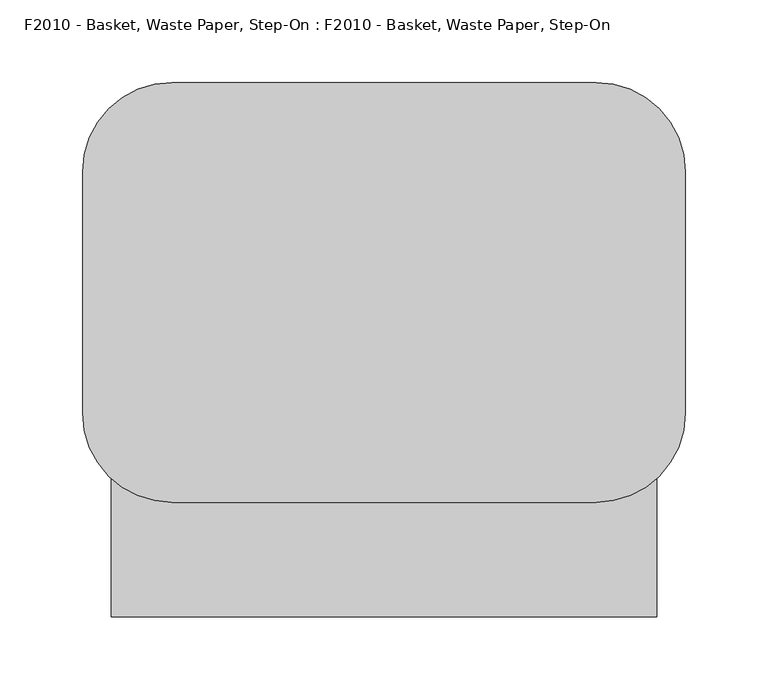
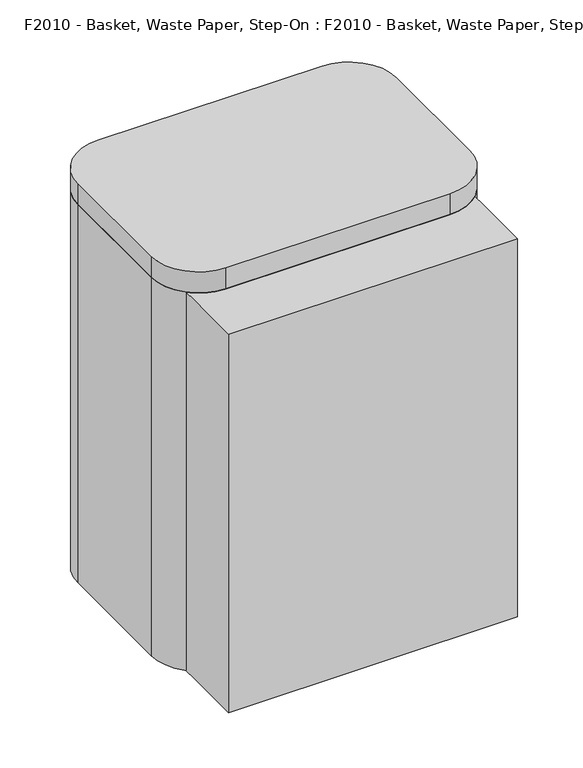
"""IFC4 building model written with IfcOpenShell, lengths in millimetres: proxy geometry, F2010 - Basket, Waste Paper, Step-On : F2010 - Basket, Waste Paper, Step-On."""

import ifcopenshell
import ifcopenshell.guid

model = None  # the IFC model being written
_history = None  # IfcOwnerHistory: only IFC2X3 demands one
_inside = {}  # id of a spatial element -> (the spatial element, [elements in it])
_under = {}  # id of a project, library or spatial element -> (it, [spatial elements below it])
_declared = {}  # id of a project -> (the project, [libraries it declares])
_typed = {}  # id of a type object -> (the type object, [elements of that type])
_made_of = {}  # id of a material, layer set ... -> (it, [elements and type objects made of it])


def new_model(schema):
    """Start an empty IFC model of exactly this schema.

    Asked for "IFC4X3", IfcOpenShell would pick the latest addendum, in which some entities
    have other attributes; the version numbers below select the first issue.
    IFC2X3 requires an IfcOwnerHistory on every rooted entity: one is made here for all.
    """
    global model, _history
    if schema == "IFC4X3":
        model = ifcopenshell.file(schema_version=(4, 3, 0, 0))
    else:
        model = ifcopenshell.file(schema=schema)
    _inside.clear()
    _under.clear()
    _declared.clear()
    _typed.clear()
    _made_of.clear()
    _history = None
    if model.schema == "IFC2X3":
        org = make("IfcOrganization", Name="unknown")
        user = make(
            "IfcPersonAndOrganization",
            ThePerson=make("IfcPerson", FamilyName="unknown"),
            TheOrganization=org,
        )
        app = make(
            "IfcApplication",
            ApplicationDeveloper=org,
            Version="unknown",
            ApplicationFullName="unknown",
            ApplicationIdentifier="unknown",
        )
        _history = make(
            "IfcOwnerHistory",
            OwningUser=user,
            OwningApplication=app,
            ChangeAction="ADDED",
            CreationDate=0,
        )
    return model


def make(cls, **values):
    """One entity of the class cls with the attributes given. An attribute that is None is left unset."""
    return model.create_entity(
        cls, **{name: value for name, value in values.items() if value is not None}
    )


def rooted(cls, **values):
    """An entity with a GlobalId (a new one), such as an element, a storey or a relation."""
    return make(cls, GlobalId=ifcopenshell.guid.new(), OwnerHistory=_history, **values)


def si_unit(unit_type, name, prefix=None):
    """IfcSIUnit, for example si_unit("LENGTHUNIT", "METRE", prefix="MILLI")."""
    return make("IfcSIUnit", UnitType=unit_type, Prefix=prefix, Name=name)


def assignment(units):
    """IfcUnitAssignment: the units of a project."""
    return None if units is None else make("IfcUnitAssignment", Units=units)


def point(xyz):
    """IfcCartesianPoint."""
    return None if xyz is None else make("IfcCartesianPoint", Coordinates=xyz)


def direction(xyz):
    """IfcDirection."""
    return None if xyz is None else make("IfcDirection", DirectionRatios=xyz)


def frame(location, z_axis=None, x_axis=None):
    """IfcAxis2Placement3D, a coordinate frame: its origin and axes. An axis left out is left unset."""
    return make(
        "IfcAxis2Placement3D",
        Location=point(location),
        Axis=direction(z_axis),
        RefDirection=direction(x_axis),
    )


def frame_2d(location, x_axis=None):
    """IfcAxis2Placement2D, a coordinate frame in the plane: its origin and x axis."""
    return make(
        "IfcAxis2Placement2D", Location=point(location), RefDirection=direction(x_axis)
    )


def origin():
    """The frame at (0, 0, 0) with its axes left unset."""
    return frame((0.0, 0.0, 0.0))


def origin_with_axes():
    """The frame at (0, 0, 0) with the z axis (0, 0, 1) and the x axis (1, 0, 0) written out."""
    return frame((0.0, 0.0, 0.0), z_axis=(0.0, 0.0, 1.0), x_axis=(1.0, 0.0, 0.0))


def place(relative_to, where):
    """IfcLocalPlacement: puts the frame where relative to a parent placement (None: the world)."""
    return make(
        "IfcLocalPlacement", PlacementRelTo=relative_to, RelativePlacement=where
    )


def context(
    kind, dimensions, precision=None, world=None, true_north=None, identifier=None
):
    """IfcGeometricRepresentationContext, for example the 3D "Model" context."""
    return make(
        "IfcGeometricRepresentationContext",
        ContextIdentifier=identifier,
        ContextType=kind,
        CoordinateSpaceDimension=dimensions,
        Precision=precision,
        WorldCoordinateSystem=world,
        TrueNorth=true_north,
    )


def project(units=None, contexts=None):
    """IfcProject with its units and contexts."""
    return rooted(
        "IfcProject",
        Name="project",
        RepresentationContexts=contexts,
        UnitsInContext=assignment(units),
    )


def spatial(cls, under=None, at=None, **own):
    """A site, building, storey or space (cls), placed at a placement, below another one or the project."""
    s = rooted(cls, ObjectPlacement=at, **own)
    if under is not None:
        _under.setdefault(under.id(), (under, []))[1].append(s)
    return s


def polyline(points):
    """IfcPolyline through the points."""
    return make("IfcPolyline", Points=[point(p) for p in points])


def circle_curve(where, radius):
    """IfcCircle in the frame where."""
    return make("IfcCircle", Position=where, Radius=radius)


def trimmed(basis, trim1, trim2, sense, master):
    """IfcTrimmedCurve: the piece of a basis curve between two trims."""
    return make(
        "IfcTrimmedCurve",
        BasisCurve=basis,
        Trim1=trim1,
        Trim2=trim2,
        SenseAgreement=sense,
        MasterRepresentation=master,
    )


def segment(curve, same_sense, transition):
    """IfcCompositeCurveSegment."""
    return make(
        "IfcCompositeCurveSegment",
        Transition=transition,
        SameSense=same_sense,
        ParentCurve=curve,
    )


def composite_curve(segments, self_intersect=None):
    """IfcCompositeCurve: segments joined end to end."""
    return make("IfcCompositeCurve", Segments=segments, SelfIntersect=self_intersect)


def outline(outer, holes=None, kind="AREA"):
    """IfcArbitraryClosedProfileDef: a profile drawn as a closed curve; with holes, ...WithVoids."""
    if holes is None:
        return make("IfcArbitraryClosedProfileDef", ProfileType=kind, OuterCurve=outer)
    return make(
        "IfcArbitraryProfileDefWithVoids",
        ProfileType=kind,
        OuterCurve=outer,
        InnerCurves=holes,
    )


def extrude(swept, where, along, depth):
    """IfcExtrudedAreaSolid: the profile swept, set in the frame where, extruded along a direction by depth."""
    return make(
        "IfcExtrudedAreaSolid",
        SweptArea=swept,
        Position=where,
        ExtrudedDirection=direction(along),
        Depth=depth,
    )


def shape(context_of_items, identifier, shape_type, items):
    """IfcShapeRepresentation: the items that make up one representation, for example the "Body"."""
    return make(
        "IfcShapeRepresentation",
        ContextOfItems=context_of_items,
        RepresentationIdentifier=identifier,
        RepresentationType=shape_type,
        Items=items,
    )


def source(mapping_origin, context_of_items, identifier, shape_type, items):
    """IfcRepresentationMap: a shape defined once, which mapped items show again and again."""
    return make(
        "IfcRepresentationMap",
        MappingOrigin=mapping_origin,
        MappedRepresentation=shape(context_of_items, identifier, shape_type, items),
    )


def transform(
    local_origin,
    x_axis=None,
    y_axis=None,
    z_axis=None,
    scale=None,
    scale2=None,
    scale3=None,
    uniform=True,
):
    """IfcCartesianTransformationOperator3D, or its non-uniform kind. x_axis, y_axis, z_axis: its Axis1, 2, 3."""
    if uniform:
        return make(
            "IfcCartesianTransformationOperator3D",
            Axis1=direction(x_axis),
            Axis2=direction(y_axis),
            LocalOrigin=point(local_origin),
            Scale=scale,
            Axis3=direction(z_axis),
        )
    return make(
        "IfcCartesianTransformationOperator3DnonUniform",
        Axis1=direction(x_axis),
        Axis2=direction(y_axis),
        LocalOrigin=point(local_origin),
        Scale=scale,
        Axis3=direction(z_axis),
        Scale2=scale2,
        Scale3=scale3,
    )


def mapped(mapping_source, mapping_target):
    """IfcMappedItem: shows the shape of a source again, moved by a transform."""
    return make(
        "IfcMappedItem", MappingSource=mapping_source, MappingTarget=mapping_target
    )


def made_of(thing, what):
    """Note that an element or type object is made of a material, layer set ...; save() writes the relation."""
    if what is not None:
        _made_of.setdefault(what.id(), (what, []))[1].append(thing)
    return thing


def element(
    cls,
    number,
    at=None,
    inside=None,
    cuts=None,
    type_object=None,
    material=None,
    context=None,
    identifier="Body",
    shape_type=None,
    held_by="IfcProductDefinitionShape",
    body=None,
    shapes=None,
    **own,
):
    """One element of the class cls, such as IfcWall. Its Tag is "e" and its number.

    at: its placement. inside: the storey or other place that contains it. cuts: it is an
    opening in that element (IfcRelVoidsElement). A single representation is given by context,
    identifier, shape_type and body (its items); several are given by shapes. held_by: the class
    of the entity that holds the representations. save() writes the other relations.
    """
    e = rooted(cls, Tag="e%d" % number, ObjectPlacement=at, **own)
    if body is not None:
        shapes = [shape(context, identifier, shape_type, body)]
    if shapes is not None:
        e.Representation = make(held_by, Representations=shapes)
    if inside is not None:
        _inside.setdefault(inside.id(), (inside, []))[1].append(e)
    if cuts is not None:
        rooted(
            "IfcRelVoidsElement", RelatingBuildingElement=cuts, RelatedOpeningElement=e
        )
    if type_object is not None:
        _typed.setdefault(type_object.id(), (type_object, []))[1].append(e)
    return made_of(e, material)


def aggregate(whole, parts):
    """IfcRelAggregates: a whole, such as a stair, and the parts it consists of."""
    return rooted("IfcRelAggregates", RelatingObject=whole, RelatedObjects=parts)


def save(model, path):
    """Write the relations noted so far, then the file.

    IfcRelAggregates (storeys below a building ...), IfcRelContainedInSpatialStructure (elements
    in a storey), IfcRelDefinesByType, IfcRelAssociatesMaterial and IfcRelDeclares: one each for
    every whole, place, type object, material and project.
    """
    for whole, parts in _under.values():
        aggregate(whole, parts)
    for where, things in _inside.values():
        rooted(
            "IfcRelContainedInSpatialStructure",
            RelatedElements=things,
            RelatingStructure=where,
        )
    for kind, things in _typed.values():
        rooted("IfcRelDefinesByType", RelatedObjects=things, RelatingType=kind)
    for what, things in _made_of.values():
        rooted("IfcRelAssociatesMaterial", RelatedObjects=things, RelatingMaterial=what)
    for by, libraries in _declared.values():
        rooted("IfcRelDeclares", RelatingContext=by, RelatedDefinitions=libraries)
    model.write(path)


def plane_surface(at):
    """IfcPlane: the flat surface through the origin of the frame at, square to its z axis."""
    return make("IfcPlane", Position=at)


def cylinder_surface(at, radius):
    """IfcCylindricalSurface: all points at the distance radius from the z axis of the frame at."""
    return make("IfcCylindricalSurface", Position=at, Radius=radius)


def revolved_surface(curve, axis_point, axis_direction):
    """IfcSurfaceOfRevolution: the curve turned about the line through axis_point along axis_direction."""
    return make(
        "IfcSurfaceOfRevolution",
        SweptCurve=make("IfcArbitraryOpenProfileDef", ProfileType="CURVE", Curve=curve),
        AxisPosition=make("IfcAxis1Placement", Location=point(axis_point), Axis=direction(axis_direction)),
    )


def advanced_brep(points, edges, surfaces, faces):
    """IfcAdvancedBrep: a solid bounded by faces that lie on surfaces and meet in shared edges.

    An edge is (start, end): straight between two places in points (the first is 0);
    or (start, end, curve); or (start, end, curve, False) where it runs against its curve.
    A face is (place in surfaces, loops), or (place, loops, False) where it looks against
    its surface's normal. A loop lists edges by number (the first is 1), with a minus sign
    where the edge is run from its end to its start. The first loop is the outer one.
    """
    corners = [point(p) for p in points]
    vertices = [make("IfcVertexPoint", VertexGeometry=c) for c in corners]
    made = []
    for start, end, *more in edges:
        made.append(
            make(
                "IfcEdgeCurve",
                EdgeStart=vertices[start],
                EdgeEnd=vertices[end],
                EdgeGeometry=more[0] if more else make("IfcPolyline", Points=[corners[start], corners[end]]),
                SameSense=more[1] if len(more) > 1 else True,
            )
        )
    hull = []
    for where, loops, *sense in faces:
        bounds = []
        for j, loop in enumerate(loops):
            ring = [make("IfcOrientedEdge", EdgeElement=made[abs(k) - 1], Orientation=k > 0) for k in loop]
            bounds.append(
                make(
                    "IfcFaceOuterBound" if j == 0 else "IfcFaceBound",
                    Bound=make("IfcEdgeLoop", EdgeList=ring),
                    Orientation=True,
                )
            )
        hull.append(make("IfcAdvancedFace", Bounds=bounds, FaceSurface=surfaces[where], SameSense=sense[0] if sense else True))
    return make("IfcAdvancedBrep", Outer=make("IfcClosedShell", CfsFaces=hull))


def f2010_basket_waste_paper_step_on_f2010_basket_waste_paper_f2c5e097(model_context):
    return source(origin(), model_context, "Body", "SolidModel", [
        advanced_brep(
        [(128.266525, 170.9615385, 457.2), (-128.266525, 170.9615385, 457.2), (-182.241525, 116.9865385, 457.2), (-182.241525, -29.0634615, 457.2), (-128.266525, -83.0384615, 457.2), (128.266525, -83.0384615, 457.2), (182.241525, -29.0634615, 457.2), (182.241525, 116.9865385, 457.2), (-114.3, 164.6115385, 457.2), (114.3, 164.6115385, 457.2), (165.1, 113.8115385, 457.2), (165.1, -25.8884615, 457.2), (114.3, -76.6884615, 457.2), (-114.3, -76.6884615, 457.2), (-165.1, -25.8884615, 457.2), (-165.1, 113.8115385, 457.2), (128.266525, 170.9615385, 0.0), (182.241525, 116.9865385, 0.0), (182.241525, -29.0634615, 0.0), (128.266525, -83.0384615, 0.0), (-128.266525, -83.0384615, 0.0), (-182.241525, -29.0634615, 0.0), (-182.241525, 116.9865385, 0.0), (-128.266525, 170.9615385, 0.0), (114.3, 164.6115385, 12.7), (-114.3, 164.6115385, 12.7), (-165.1, 113.8115385, 12.7), (-165.1, -25.8884615, 12.7), (-114.3, -76.6884615, 12.7), (114.3, -76.6884615, 12.7), (165.1, -25.8884615, 12.7), (165.1, 113.8115385, 12.7)],
        [
            (0, 1),
            (1, 2, circle_curve(frame((-128.266525, 116.9865385, 457.2), z_axis=(0.0, 0.0, 1.0), x_axis=(1.0, 0.0, 0.0)), 53.975)),
            (2, 3),
            (3, 4, circle_curve(frame((-128.266525, -29.0634615, 457.2), z_axis=(0.0, 0.0, 1.0), x_axis=(1.0, 0.0, 0.0)), 53.975)),
            (4, 5),
            (5, 6, circle_curve(frame((128.266525, -29.0634615, 457.2), z_axis=(0.0, 0.0, 1.0), x_axis=(1.0, 0.0, 0.0)), 53.975)),
            (6, 7),
            (7, 0, circle_curve(frame((128.266525, 116.9865385, 457.2), z_axis=(0.0, 0.0, 1.0), x_axis=(1.0, 0.0, 0.0)), 53.975)),
            (8, 9),
            (9, 10, circle_curve(frame((114.3, 113.8115385, 457.2), z_axis=(0.0, 0.0, -1.0), x_axis=(1.0, 0.0, 0.0)), 50.8)),
            (10, 11),
            (11, 12, circle_curve(frame((114.3, -25.8884615, 457.2), z_axis=(0.0, 0.0, -1.0), x_axis=(1.0, 0.0, 0.0)), 50.8)),
            (12, 13),
            (13, 14, circle_curve(frame((-114.3, -25.8884615, 457.2), z_axis=(0.0, 0.0, -1.0), x_axis=(1.0, 0.0, 0.0)), 50.8)),
            (14, 15),
            (15, 8, circle_curve(frame((-114.3, 113.8115385, 457.2), z_axis=(0.0, 0.0, -1.0), x_axis=(1.0, 0.0, 0.0)), 50.8)),
            (16, 17, circle_curve(frame((128.266525, 116.9865385, 0.0), z_axis=(0.0, 0.0, -1.0), x_axis=(1.0, 0.0, 0.0)), 53.975)),
            (17, 18),
            (18, 19, circle_curve(frame((128.266525, -29.0634615, 0.0), z_axis=(0.0, 0.0, -1.0), x_axis=(1.0, 0.0, 0.0)), 53.975)),
            (19, 20),
            (20, 21, circle_curve(frame((-128.266525, -29.0634615, 0.0), z_axis=(0.0, 0.0, -1.0), x_axis=(1.0, 0.0, 0.0)), 53.975)),
            (21, 22),
            (22, 23, circle_curve(frame((-128.266525, 116.9865385, 0.0), z_axis=(0.0, 0.0, -1.0), x_axis=(1.0, 0.0, 0.0)), 53.975)),
            (23, 16),
            (0, 16),
            (23, 1),
            (22, 2),
            (21, 3),
            (20, 4),
            (19, 5),
            (18, 6),
            (17, 7),
            (24, 25),
            (25, 26, circle_curve(frame((-114.3, 113.8115385, 12.7), z_axis=(0.0, 0.0, 1.0), x_axis=(1.0, 0.0, 0.0)), 50.8)),
            (26, 27),
            (27, 28, circle_curve(frame((-114.3, -25.8884615, 12.7), z_axis=(0.0, 0.0, 1.0), x_axis=(1.0, 0.0, 0.0)), 50.8)),
            (28, 29),
            (29, 30, circle_curve(frame((114.3, -25.8884615, 12.7), z_axis=(0.0, 0.0, 1.0), x_axis=(1.0, 0.0, 0.0)), 50.8)),
            (30, 31),
            (31, 24, circle_curve(frame((114.3, 113.8115385, 12.7), z_axis=(0.0, 0.0, 1.0), x_axis=(1.0, 0.0, 0.0)), 50.8)),
            (24, 9),
            (8, 25),
            (15, 26),
            (14, 27),
            (13, 28),
            (12, 29),
            (11, 30),
            (10, 31),
        ],
        [
            plane_surface(frame((-182.241525, 170.9615385, 457.2), z_axis=(0.0, 0.0, 1.0), x_axis=(-1.0, 0.0, 0.0))),
            plane_surface(frame((-182.241525, 170.9615385, 0.0), z_axis=(0.0, 0.0, -1.0), x_axis=(1.0, 0.0, 0.0))),
            plane_surface(frame((128.266525, 170.9615385, 457.2), z_axis=(0.0, 1.0, 0.0), x_axis=(0.0, 0.0, -1.0))),
            cylinder_surface(frame((-128.266525, 116.9865385, 0.0), z_axis=(0.0, 0.0, 1.0), x_axis=(1.0, 0.0, 0.0)), 53.975),
            plane_surface(frame((-182.241525, 116.9865385, 457.2), z_axis=(-1.0, 0.0, 0.0), x_axis=(0.0, 0.0, -1.0))),
            cylinder_surface(frame((-128.266525, -29.0634615, 0.0), z_axis=(0.0, 0.0, 1.0), x_axis=(1.0, 0.0, 0.0)), 53.975),
            plane_surface(frame((-128.266525, -83.0384615, 457.2), z_axis=(0.0, -1.0, 0.0), x_axis=(0.0, 0.0, -1.0))),
            cylinder_surface(frame((128.266525, -29.0634615, 0.0), z_axis=(0.0, 0.0, 1.0), x_axis=(1.0, 0.0, 0.0)), 53.975),
            plane_surface(frame((182.241525, -29.0634615, 457.2), z_axis=(1.0, 0.0, 0.0), x_axis=(0.0, 0.0, -1.0))),
            cylinder_surface(frame((128.266525, 116.9865385, 0.0), z_axis=(0.0, 0.0, 1.0), x_axis=(1.0, 0.0, 0.0)), 53.975),
            plane_surface(frame((-125.091525, 164.6115385, 12.7), z_axis=(0.0, 0.0, 1.0), x_axis=(1.0, 0.0, 0.0))),
            plane_surface(frame((114.3, 164.6115385, 457.2), z_axis=(0.0, -1.0, 0.0), x_axis=(0.0, 0.0, -1.0))),
            revolved_surface(polyline([(-63.5, 113.8115385, 457.2), (-63.5, 113.8115385, 12.7)]), (-114.3, 113.8115385, 12.7), (0.0, 0.0, 1.0)),
            plane_surface(frame((-165.1, 113.8115385, 457.2), z_axis=(1.0, 0.0, 0.0), x_axis=(0.0, 0.0, -1.0))),
            revolved_surface(polyline([(-63.5, -25.8884615, 457.2), (-63.5, -25.8884615, 12.7)]), (-114.3, -25.8884615, 12.7), (0.0, 0.0, 1.0)),
            plane_surface(frame((-114.3, -76.6884615, 457.2), z_axis=(0.0, 1.0, 0.0), x_axis=(0.0, 0.0, -1.0))),
            revolved_surface(polyline([(165.1, -25.8884615, 457.2), (165.1, -25.8884615, 12.7)]), (114.3, -25.8884615, 12.7), (0.0, 0.0, 1.0)),
            plane_surface(frame((165.1, -25.8884615, 457.2), z_axis=(-1.0, 0.0, 0.0), x_axis=(0.0, 0.0, -1.0))),
            revolved_surface(polyline([(165.1, 113.8115385, 457.2), (165.1, 113.8115385, 12.7)]), (114.3, 113.8115385, 12.7), (0.0, 0.0, 1.0)),
        ],
        [
            (0, [[1, 2, 3, 4, 5, 6, 7, 8], [9, 10, 11, 12, 13, 14, 15, 16]]),
            (1, [[17, 18, 19, 20, 21, 22, 23, 24]]),
            (2, [[-1, 25, -24, 26]]),
            (3, [[-2, -26, -23, 27]]),
            (4, [[-3, -27, -22, 28]]),
            (5, [[-4, -28, -21, 29]]),
            (6, [[-5, -29, -20, 30]]),
            (7, [[-6, -30, -19, 31]]),
            (8, [[-7, -31, -18, 32]]),
            (9, [[-8, -32, -17, -25]]),
            (10, [[33, 34, 35, 36, 37, 38, 39, 40]]),
            (11, [[-33, 41, -9, 42]]),
            (12, [[-34, -42, -16, 43]]),
            (13, [[-35, -43, -15, 44]]),
            (14, [[-36, -44, -14, 45]]),
            (15, [[-37, -45, -13, 46]]),
            (16, [[-38, -46, -12, 47]]),
            (17, [[-39, -47, -11, 48]]),
            (18, [[-40, -48, -10, -41]]),
        ],
    ),
        extrude(outline(polyline([(50.8, -83.0384615), (-50.8, -83.0384615), (-50.8, -6.8384615), (50.8, -6.8384615), (50.8, -83.0384615)])), origin_with_axes(), (0.0, 0.0, 1.0), 105.5317808),
        extrude(outline(polyline([(38.1, -57.6384615), (38.1, -133.8384615), (-38.1, -133.8384615), (-38.1, -57.6384615), (38.1, -57.6384615)])), origin_with_axes(), (0.0, 0.0, 1.0), 50.8),
        extrude(outline(composite_curve([segment(trimmed(circle_curve(frame_2d((128.266525, 116.9865385)), 53.975), [point((128.266525, 170.9615385))], [point((182.241525, 116.9865385))], False, "CARTESIAN"), True, "CONTINUOUS"), segment(polyline([(182.241525, 116.9865385), (182.241525, -29.0634615)]), True, "CONTINUOUS"), segment(trimmed(circle_curve(frame_2d((128.266525, -29.0634615)), 53.975), [point((182.241525, -29.0634615))], [point((128.266525, -83.0384615))], False, "CARTESIAN"), True, "CONTINUOUS"), segment(polyline([(128.266525, -83.0384615), (-128.266525, -83.0384615)]), True, "CONTINUOUS"), segment(trimmed(circle_curve(frame_2d((-128.266525, -29.0634615)), 53.975), [point((-128.266525, -83.0384615))], [point((-182.241525, -29.0634615))], False, "CARTESIAN"), True, "CONTINUOUS"), segment(polyline([(-182.241525, -29.0634615), (-182.241525, 116.9865385)]), True, "CONTINUOUS"), segment(trimmed(circle_curve(frame_2d((-128.266525, 116.9865385)), 53.975), [point((-182.241525, 116.9865385))], [point((-128.266525, 170.9615385))], False, "CARTESIAN"), True, "CONTINUOUS"), segment(polyline([(-128.266525, 170.9615385), (128.266525, 170.9615385)]), True, "CONTINUOUS")], self_intersect=False)), frame((0.0, 0.0, 457.2), z_axis=(0.0, 0.0, 1.0), x_axis=(1.0, 0.0, 0.0)), (0.0, 0.0, 1.0), 25.4),
        extrude(outline(polyline([(-165.1, 152.4), (165.1, 152.4), (165.1, -152.4), (-165.1, -152.4), (-165.1, 0.0), (-165.1, 152.4)])), origin_with_axes(), (0.0, 0.0, 1.0), 457.2),
    ])


if __name__ == "__main__":
    model = new_model("IFC4")
    model_context = context("Model", 3, world=origin())
    ifc_project = project(units=[si_unit("LENGTHUNIT", "METRE", prefix="MILLI")], contexts=[model_context])
    site = spatial("IfcSite", under=ifc_project)
    building = spatial("IfcBuilding", under=site)
    placement = place(None, origin())
    f2010_basket_waste_paper_step_on_f2010_basket_waste_paper_shape = f2010_basket_waste_paper_step_on_f2010_basket_waste_paper_f2c5e097(model_context)
    element("IfcBuildingElementProxy", 1, Name="F2010 - Basket, Waste Paper, Step-On : F2010 - Basket, Waste Paper, Step-On", ObjectType="F2010 - Basket, Waste Paper, Step-On : F2010 - Basket, Waste Paper, Step-On", at=placement, inside=building, context=model_context, shape_type="MappedRepresentation", body=[
        mapped(f2010_basket_waste_paper_step_on_f2010_basket_waste_paper_shape, transform((0.0, 0.0, 0.0), x_axis=(1.0, 0.0, 0.0), y_axis=(0.0, 1.0, 0.0), z_axis=(0.0, 0.0, 1.0))),
    ])
    save(model, "model.ifc")

# Revit data of these elements
# Type "F2010 - Basket, Waste Paper, Step-On : F2010 - Basket, Waste Paper, Step-On"
#   Watts2 = "0"
#   Watts1 = "0"
#   Unit_Issue = "EA"
#   UTIL_6_Misc = "-"
#   UTIL_5_NonMedGas = "-"
#   UTIL_4_MiscGas = "-"
#   UTIL_3_MedGas = "-"
#   UTIL_2_Elec = "-"
#   UTIL_1_WaterDrain = "-"
#   Nomenclature = "Basket, Wastepaper, Step-On"
#   NSN = "7240007883953"
#   Location [instance default] = ""
#   JSN = "F2010"
#   Fund_Source_VA = "-"
#   Fund_Source_Navy = "-"
#   Fund_Source_Army = "-"
#   Fund_Source_AF = "-"
#   ELEC_Volts2 = "0"
#   ELEC_Volts1 = "0"
#   ELEC_Phase2 = "0"
#   ELEC_Phase1 = "0"
#   ELEC_HertzSwitch = "0"
#   ELEC_HertzDependent = "0"
#   ELEC_Hertz = "0"
#   ELEC_Amps2 = "0"
#   ELEC_Amps1 = "0"
#   DetailDescription = "\"Step-on\" wastepaper basket with inner liner and foot petal activated flip top."
#   CAT_VA = "C"
#   CAT_Navy = "C"
#   CAT_IHS = "-"
#   CAT_Army = "C"
#   CAT_AF = "C"
#   BTUperhour = "0"
#   Weight_IP = 12
#   DIM_Width_IP = 1' - 1"
#   DIM_Height_IP = 1' - 6"
#   DIM_Depth_IP = 1' - 0"
# Element 1 (IfcBuildingElementProxy, "F2010 - Basket, Waste Paper, Step-On : F2010 - Basket, Waste Paper, Step-On")
#   Location = "TLTS2"
#   Materials on its faces: "Metal - Chrome", "EquipSpace"
# Materials
#   "Metal - Chrome": class "Metal", colour RGB 17 17 17, transparency 0
#   "EquipSpace": class "Unassigned", colour RGB 221 217 195, transparency 0.5
